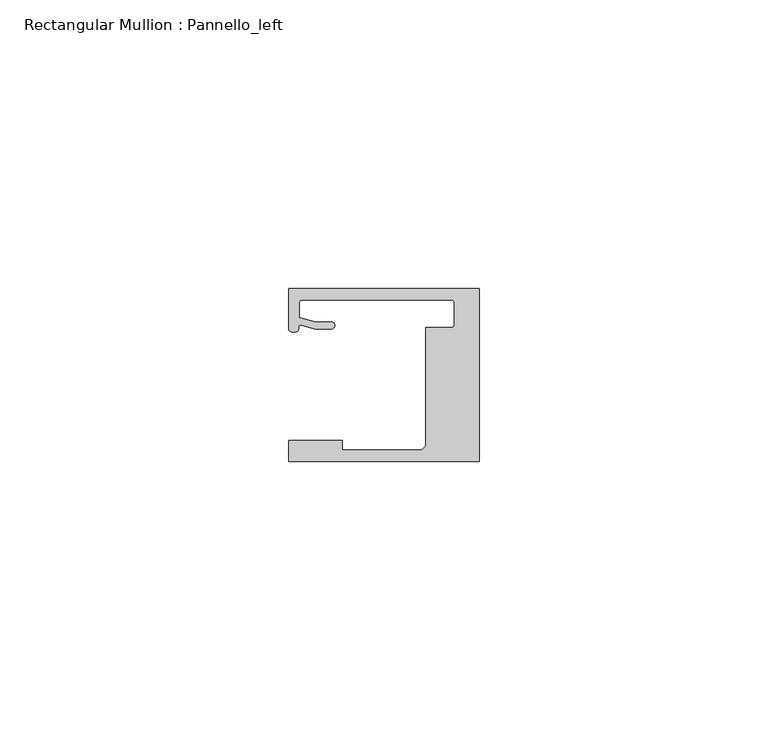
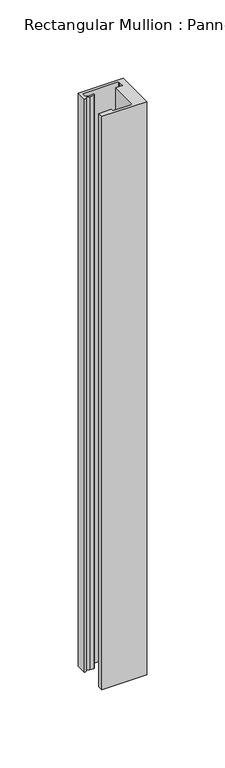
"""IFC4 building model written with IfcOpenShell, lengths in millimetres: member geometry, Rectangular Mullion : Pannello_left."""

from ifc_helpers import new_model, si_unit, frame, origin, place, context, project, spatial, polyline, circle_curve, source, transform, mapped, element, save
from ifc_brep_helpers import plane_surface, cylinder_surface, revolved_surface, extruded_surface, spline_curve, advanced_brep


def rectangular_mullion_pannello_left_8b5c6db7(model_context):
    return source(origin(), model_context, "Body", "AdvancedBrep", [
        advanced_brep(
        [(-33.0, -15.0, 0.0), (0.0, -15.0, 0.0), (0.0, 15.0, 0.0), (-33.0000135, 15.0, 0.0), (-33.0000135, 8.0000472, 0.0), (-30.9223017, 8.6490241, 0.0), (-28.4999305, 7.9999523, 0.0), (-25.59998, 7.9999523, 0.0), (-25.59998, 9.1999523, 0.0), (-28.3419477, 9.1999523, 0.0), (-31.19998, 9.9657591, 0.0), (-31.19998, 12.50001, 0.0), (-30.69998, 13.00001, 0.0), (-4.7999726, 13.00001, 0.0), (-4.2999726, 12.50001, 0.0), (-4.2999726, 8.7500595, 0.0), (-4.7999726, 8.2500595, 0.0), (-9.2999726, 8.2500595, 0.0), (-9.2999726, -12.2999849, 0.0), (-10.0000103, -13.0000004, 0.0), (-23.700041, -13.0000004, 0.0), (-23.700041, -11.3000004, 0.0), (-33.0, -11.3000004, 0.0), (-33.0, -15.0, -446.9999865), (-33.0, -11.3000004, -446.9999865), (-23.700041, -11.3000004, -446.9999865), (-23.700041, -13.0000004, -446.9999865), (-10.0000103, -13.0000004, -446.9999865), (-9.2999726, -12.2999849, -446.9999865), (-9.2999726, 8.2500595, -446.9999865), (-4.7999726, 8.2500595, -446.9999865), (-4.2999726, 8.7500595, -446.9999865), (-4.2999726, 12.50001, -446.9999865), (-4.7999726, 13.00001, -446.9999865), (-30.69998, 13.00001, -446.9999865), (-31.19998, 12.50001, -446.9999865), (-31.19998, 9.9657591, -446.9999865), (-28.3419477, 9.1999523, -446.9999865), (-25.59998, 9.1999523, -446.9999865), (-25.59998, 7.9999523, -446.9999865), (-28.4999305, 7.9999523, -446.9999865), (-30.9223017, 8.6490241, -446.9999865), (-33.0000135, 8.0000472, -446.9999865), (-33.0000135, 15.0, -446.9999865), (0.0, 15.0, -446.9999865), (0.0, -15.0, -446.9999865)],
        [
            (0, 1),
            (1, 2),
            (2, 3),
            (3, 4),
            (4, 5, spline_curve(3, [(-33.0000135, 8.0000472, 0.0), (-33.0000135, 7.457047519, 0.0), (-32.262327879, 7.456527435, 0.0), (-31.357433266, 7.563996614, 0.0), (-31.305645054, 7.690065204, 0.0), (-31.298563602, 8.366228555, 0.0), (-31.312054066, 8.717747958, 0.0), (-30.9223017, 8.6490241, 0.0)], [4, 2, 2, 4], [0.0, 0.0027053965905959043, 0.0058611956533709, 0.007702013405570312])),
            (5, 6),
            (6, 7),
            (7, 8, circle_curve(frame((-25.59998, 8.5999523, 0.0), z_axis=(0.0, 0.0, 1.0), x_axis=(0.0, 1.0, 0.0)), 0.6)),
            (8, 9),
            (9, 10),
            (10, 11),
            (11, 12, circle_curve(frame((-30.69998, 12.50001, 0.0), z_axis=(0.0, 0.0, -1.0), x_axis=(0.0, 1.0, 0.0)), 0.5)),
            (12, 13),
            (13, 14, circle_curve(frame((-4.7999726, 12.50001, 0.0), z_axis=(0.0, 0.0, -1.0), x_axis=(1.0, 0.0, 0.0)), 0.5)),
            (14, 15),
            (15, 16, circle_curve(frame((-4.7999726, 8.7500595, 0.0), z_axis=(0.0, 0.0, -1.0), x_axis=(0.0, -1.0, 0.0)), 0.5)),
            (16, 17),
            (17, 18),
            (18, 19),
            (19, 20),
            (20, 21),
            (21, 22),
            (22, 0),
            (23, 24),
            (24, 25),
            (25, 26),
            (26, 27),
            (27, 28),
            (28, 29),
            (29, 30),
            (30, 31, circle_curve(frame((-4.7999726, 8.7500595, -446.9999865), z_axis=(0.0, 0.0, 1.0), x_axis=(0.0, -1.0, 0.0)), 0.5)),
            (31, 32),
            (32, 33, circle_curve(frame((-4.7999726, 12.50001, -446.9999865), z_axis=(0.0, 0.0, 1.0), x_axis=(1.0, 0.0, 0.0)), 0.5)),
            (33, 34),
            (34, 35, circle_curve(frame((-30.69998, 12.50001, -446.9999865), z_axis=(0.0, 0.0, 1.0), x_axis=(0.0, 1.0, 0.0)), 0.5)),
            (35, 36),
            (36, 37),
            (37, 38),
            (38, 39, circle_curve(frame((-25.59998, 8.5999523, -446.9999865), z_axis=(0.0, 0.0, -1.0), x_axis=(0.0, 1.0, 0.0)), 0.6)),
            (39, 40),
            (40, 41),
            (41, 42, spline_curve(3, [(-30.9223017, 8.6490241, -446.9999865), (-31.312054066, 8.717747958, -446.9999865), (-31.298563602, 8.366228555, -446.9999865), (-31.305645054, 7.690065204, -446.9999865), (-31.357433266, 7.563996614, -446.9999865), (-32.262327879, 7.456527435, -446.9999865), (-33.0000135, 7.457047519, -446.9999865), (-33.0000135, 8.0000472, -446.9999865)], [4, 2, 2, 4], [0.0, 0.001840817752199412, 0.004996616814974408, 0.007702013405570312])),
            (42, 43),
            (43, 44),
            (44, 45),
            (45, 23),
            (0, 23),
            (45, 1),
            (44, 2),
            (43, 3),
            (42, 4),
            (41, 5),
            (40, 6),
            (39, 7),
            (38, 8),
            (37, 9),
            (36, 10),
            (35, 11),
            (34, 12),
            (33, 13),
            (32, 14),
            (31, 15),
            (30, 16),
            (29, 17),
            (28, 18),
            (27, 19),
            (26, 20),
            (25, 21),
            (24, 22),
        ],
        [
            plane_surface(frame((0.0, -36.2491502, 0.0), z_axis=(0.0, 0.0, 1.0), x_axis=(-1.0, 0.0, 0.0))),
            plane_surface(frame((0.0, -36.2491502, -446.9999865), z_axis=(0.0, 0.0, -1.0), x_axis=(-1.0, 0.0, 0.0))),
            plane_surface(frame((-33.0, -15.0, 0.0), z_axis=(0.0, -1.0, 0.0), x_axis=(0.0, 0.0, -1.0))),
            plane_surface(frame((0.0, -15.0, 0.0), z_axis=(1.0, 0.0, 0.0), x_axis=(0.0, 0.0, -1.0))),
            plane_surface(frame((0.0, 15.0, 0.0), z_axis=(0.0, 1.0, 0.0), x_axis=(0.0, 0.0, -1.0))),
            plane_surface(frame((-33.0000135, 15.0, 0.0), z_axis=(-1.0, 0.0, 0.0), x_axis=(0.0, 0.0, -1.0))),
            extruded_surface(spline_curve(3, [(-33.0000135, 8.0000472, -446.9999865), (-33.0000135, 7.457047519, -446.9999865), (-32.262327879, 7.456527435, -446.9999865), (-31.357433266, 7.563996614, -446.9999865), (-31.305645054, 7.690065204, -446.9999865), (-31.298563602, 8.366228555, -446.9999865), (-31.312054066, 8.717747958, -446.9999865), (-30.9223017, 8.6490241, -446.9999865)], [4, 2, 2, 4], [0.0, 0.0027053965905959043, 0.0058611956533709, 0.007702013405570312]), (0.0, 0.0, 446.9999865), 446.9999865),
            plane_surface(frame((-30.9223017, 8.6490241, 0.0), z_axis=(-0.25881883200192934, -0.9659258833891746, 0.0), x_axis=(0.0, 0.0, -1.0))),
            plane_surface(frame((-28.4999305, 7.9999523, 0.0), z_axis=(0.0, -1.0, 0.0), x_axis=(0.0, 0.0, -1.0))),
            cylinder_surface(frame((-25.59998, 8.5999523, 0.0), z_axis=(0.0, 0.0, 1.0), x_axis=(0.0, 1.0, 0.0)), 0.6),
            plane_surface(frame((-25.59998, 9.1999523, 0.0), z_axis=(0.0, 1.0, 0.0), x_axis=(0.0, 0.0, -1.0))),
            plane_surface(frame((-28.3419477, 9.1999523, 0.0), z_axis=(0.25881883204288636, 0.9659258833782002, 0.0), x_axis=(0.0, 0.0, -1.0))),
            plane_surface(frame((-31.19998, 9.9657591, 0.0), z_axis=(1.0, 0.0, 0.0), x_axis=(0.0, 0.0, -1.0))),
            revolved_surface(polyline([(-30.69998, 13.00001, -446.9999865), (-30.69998, 13.00001, 0.0)]), (-30.69998, 12.50001, 0.0), (0.0, 0.0, -1.0)),
            plane_surface(frame((-30.69998, 13.00001, 0.0), z_axis=(0.0, -1.0, 0.0), x_axis=(0.0, 0.0, -1.0))),
            revolved_surface(polyline([(-4.2999726, 12.50001, -446.9999865), (-4.2999726, 12.50001, 0.0)]), (-4.7999726, 12.50001, 0.0), (0.0, 0.0, -1.0)),
            plane_surface(frame((-4.2999726, 12.50001, 0.0), z_axis=(-1.0, 0.0, 0.0), x_axis=(0.0, 0.0, -1.0))),
            revolved_surface(polyline([(-4.7999726, 8.2500595, -446.9999865), (-4.7999726, 8.2500595, 0.0)]), (-4.7999726, 8.7500595, 0.0), (0.0, 0.0, -1.0)),
            plane_surface(frame((-4.7999726, 8.2500595, 0.0), z_axis=(0.0, 1.0, 0.0), x_axis=(0.0, 0.0, -1.0))),
            plane_surface(frame((-9.2999726, 8.2500595, 0.0), z_axis=(-1.0, 0.0, 0.0), x_axis=(0.0, 0.0, -1.0))),
            plane_surface(frame((-9.2999726, -12.2999849, 0.0), z_axis=(-0.7070955486277984, 0.7071180135668678, 0.0), x_axis=(0.0, 0.0, -1.0))),
            plane_surface(frame((-10.0000103, -13.0000004, 0.0), z_axis=(0.0, 1.0, 0.0), x_axis=(0.0, 0.0, -1.0))),
            plane_surface(frame((-23.700041, -13.0000004, 0.0), z_axis=(1.0, 0.0, 0.0), x_axis=(0.0, 0.0, -1.0))),
            plane_surface(frame((-23.700041, -11.3000004, 0.0), z_axis=(0.0, 1.0, 0.0), x_axis=(0.0, 0.0, -1.0))),
            plane_surface(frame((-33.0, -11.3000004, 0.0), z_axis=(-1.0, 0.0, 0.0), x_axis=(0.0, 0.0, -1.0))),
        ],
        [
            (0, [[1, 2, 3, 4, 5, 6, 7, 8, 9, 10, 11, 12, 13, 14, 15, 16, 17, 18, 19, 20, 21, 22, 23]]),
            (1, [[24, 25, 26, 27, 28, 29, 30, 31, 32, 33, 34, 35, 36, 37, 38, 39, 40, 41, 42, 43, 44, 45, 46]]),
            (2, [[-1, 47, -46, 48]]),
            (3, [[-2, -48, -45, 49]]),
            (4, [[-3, -49, -44, 50]]),
            (5, [[-4, -50, -43, 51]]),
            (6, [[-5, -51, -42, 52]]),
            (7, [[-6, -52, -41, 53]]),
            (8, [[-7, -53, -40, 54]]),
            (9, [[-8, -54, -39, 55]]),
            (10, [[-9, -55, -38, 56]]),
            (11, [[-10, -56, -37, 57]]),
            (12, [[-11, -57, -36, 58]]),
            (13, [[-12, -58, -35, 59]]),
            (14, [[-13, -59, -34, 60]]),
            (15, [[-14, -60, -33, 61]]),
            (16, [[-15, -61, -32, 62]]),
            (17, [[-16, -62, -31, 63]]),
            (18, [[-17, -63, -30, 64]]),
            (19, [[-18, -64, -29, 65]]),
            (20, [[-19, -65, -28, 66]]),
            (21, [[-20, -66, -27, 67]]),
            (22, [[-21, -67, -26, 68]]),
            (23, [[-22, -68, -25, 69]]),
            (24, [[-23, -69, -24, -47]]),
        ],
    ),
    ])


if __name__ == "__main__":
    model = new_model("IFC4")
    model_context = context("Model", 3, world=origin())
    ifc_project = project(units=[si_unit("LENGTHUNIT", "METRE", prefix="MILLI")], contexts=[model_context])
    site = spatial("IfcSite", under=ifc_project)
    building = spatial("IfcBuilding", under=site)
    placement = place(None, origin())
    rectangular_mullion_pannello_left_shape = rectangular_mullion_pannello_left_8b5c6db7(model_context)
    element("IfcMember", 1, ObjectType="Rectangular Mullion : Pannello_left", at=placement, inside=building, context=model_context, shape_type="MappedRepresentation", body=[
        mapped(rectangular_mullion_pannello_left_shape, transform((0.0, 0.0, 0.0), x_axis=(1.0, 0.0, 0.0), y_axis=(0.0, 1.0, 0.0), z_axis=(0.0, 0.0, 1.0))),
    ])
    save(model, "model.ifc")

# Revit data of these elements
# Type "Rectangular Mullion : Pannello_left"
#   built-in parameter 1007322 = 0.0984252 (stored number, unit not read)
#   built-in parameter 1007320 = 0.0305117 (stored number, unit not read)
